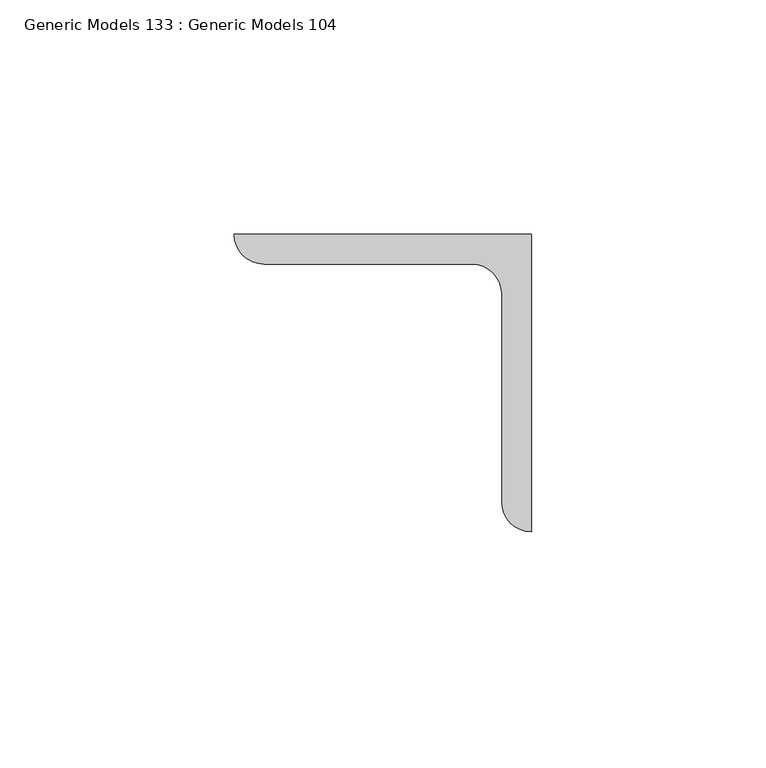
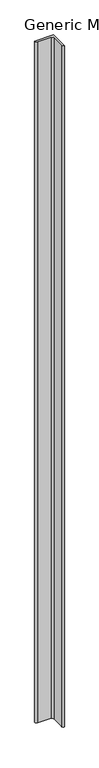
"""IFC4 building model written with IfcOpenShell, lengths in millimetres: proxy geometry, Generic Models 133 : Generic Models 104."""

import ifcopenshell
import ifcopenshell.guid

model = None  # the IFC model being written
_history = None  # IfcOwnerHistory: only IFC2X3 demands one
_inside = {}  # id of a spatial element -> (the spatial element, [elements in it])
_under = {}  # id of a project, library or spatial element -> (it, [spatial elements below it])
_declared = {}  # id of a project -> (the project, [libraries it declares])
_typed = {}  # id of a type object -> (the type object, [elements of that type])
_made_of = {}  # id of a material, layer set ... -> (it, [elements and type objects made of it])


def new_model(schema):
    """Start an empty IFC model of exactly this schema.

    Asked for "IFC4X3", IfcOpenShell would pick the latest addendum, in which some entities
    have other attributes; the version numbers below select the first issue.
    IFC2X3 requires an IfcOwnerHistory on every rooted entity: one is made here for all.
    """
    global model, _history
    if schema == "IFC4X3":
        model = ifcopenshell.file(schema_version=(4, 3, 0, 0))
    else:
        model = ifcopenshell.file(schema=schema)
    _inside.clear()
    _under.clear()
    _declared.clear()
    _typed.clear()
    _made_of.clear()
    _history = None
    if model.schema == "IFC2X3":
        org = make("IfcOrganization", Name="unknown")
        user = make(
            "IfcPersonAndOrganization",
            ThePerson=make("IfcPerson", FamilyName="unknown"),
            TheOrganization=org,
        )
        app = make(
            "IfcApplication",
            ApplicationDeveloper=org,
            Version="unknown",
            ApplicationFullName="unknown",
            ApplicationIdentifier="unknown",
        )
        _history = make(
            "IfcOwnerHistory",
            OwningUser=user,
            OwningApplication=app,
            ChangeAction="ADDED",
            CreationDate=0,
        )
    return model


def make(cls, **values):
    """One entity of the class cls with the attributes given. An attribute that is None is left unset."""
    return model.create_entity(
        cls, **{name: value for name, value in values.items() if value is not None}
    )


def rooted(cls, **values):
    """An entity with a GlobalId (a new one), such as an element, a storey or a relation."""
    return make(cls, GlobalId=ifcopenshell.guid.new(), OwnerHistory=_history, **values)


def si_unit(unit_type, name, prefix=None):
    """IfcSIUnit, for example si_unit("LENGTHUNIT", "METRE", prefix="MILLI")."""
    return make("IfcSIUnit", UnitType=unit_type, Prefix=prefix, Name=name)


def assignment(units):
    """IfcUnitAssignment: the units of a project."""
    return None if units is None else make("IfcUnitAssignment", Units=units)


def point(xyz):
    """IfcCartesianPoint."""
    return None if xyz is None else make("IfcCartesianPoint", Coordinates=xyz)


def direction(xyz):
    """IfcDirection."""
    return None if xyz is None else make("IfcDirection", DirectionRatios=xyz)


def frame(location, z_axis=None, x_axis=None):
    """IfcAxis2Placement3D, a coordinate frame: its origin and axes. An axis left out is left unset."""
    return make(
        "IfcAxis2Placement3D",
        Location=point(location),
        Axis=direction(z_axis),
        RefDirection=direction(x_axis),
    )


def frame_2d(location, x_axis=None):
    """IfcAxis2Placement2D, a coordinate frame in the plane: its origin and x axis."""
    return make(
        "IfcAxis2Placement2D", Location=point(location), RefDirection=direction(x_axis)
    )


def origin():
    """The frame at (0, 0, 0) with its axes left unset."""
    return frame((0.0, 0.0, 0.0))


def place(relative_to, where):
    """IfcLocalPlacement: puts the frame where relative to a parent placement (None: the world)."""
    return make(
        "IfcLocalPlacement", PlacementRelTo=relative_to, RelativePlacement=where
    )


def context(
    kind, dimensions, precision=None, world=None, true_north=None, identifier=None
):
    """IfcGeometricRepresentationContext, for example the 3D "Model" context."""
    return make(
        "IfcGeometricRepresentationContext",
        ContextIdentifier=identifier,
        ContextType=kind,
        CoordinateSpaceDimension=dimensions,
        Precision=precision,
        WorldCoordinateSystem=world,
        TrueNorth=true_north,
    )


def project(units=None, contexts=None):
    """IfcProject with its units and contexts."""
    return rooted(
        "IfcProject",
        Name="project",
        RepresentationContexts=contexts,
        UnitsInContext=assignment(units),
    )


def spatial(cls, under=None, at=None, **own):
    """A site, building, storey or space (cls), placed at a placement, below another one or the project."""
    s = rooted(cls, ObjectPlacement=at, **own)
    if under is not None:
        _under.setdefault(under.id(), (under, []))[1].append(s)
    return s


def polyline(points):
    """IfcPolyline through the points."""
    return make("IfcPolyline", Points=[point(p) for p in points])


def circle_curve(where, radius):
    """IfcCircle in the frame where."""
    return make("IfcCircle", Position=where, Radius=radius)


def trimmed(basis, trim1, trim2, sense, master):
    """IfcTrimmedCurve: the piece of a basis curve between two trims."""
    return make(
        "IfcTrimmedCurve",
        BasisCurve=basis,
        Trim1=trim1,
        Trim2=trim2,
        SenseAgreement=sense,
        MasterRepresentation=master,
    )


def segment(curve, same_sense, transition):
    """IfcCompositeCurveSegment."""
    return make(
        "IfcCompositeCurveSegment",
        Transition=transition,
        SameSense=same_sense,
        ParentCurve=curve,
    )


def composite_curve(segments, self_intersect=None):
    """IfcCompositeCurve: segments joined end to end."""
    return make("IfcCompositeCurve", Segments=segments, SelfIntersect=self_intersect)


def outline(outer, holes=None, kind="AREA"):
    """IfcArbitraryClosedProfileDef: a profile drawn as a closed curve; with holes, ...WithVoids."""
    if holes is None:
        return make("IfcArbitraryClosedProfileDef", ProfileType=kind, OuterCurve=outer)
    return make(
        "IfcArbitraryProfileDefWithVoids",
        ProfileType=kind,
        OuterCurve=outer,
        InnerCurves=holes,
    )


def extrude(swept, where, along, depth):
    """IfcExtrudedAreaSolid: the profile swept, set in the frame where, extruded along a direction by depth."""
    return make(
        "IfcExtrudedAreaSolid",
        SweptArea=swept,
        Position=where,
        ExtrudedDirection=direction(along),
        Depth=depth,
    )


def shape(context_of_items, identifier, shape_type, items):
    """IfcShapeRepresentation: the items that make up one representation, for example the "Body"."""
    return make(
        "IfcShapeRepresentation",
        ContextOfItems=context_of_items,
        RepresentationIdentifier=identifier,
        RepresentationType=shape_type,
        Items=items,
    )


def source(mapping_origin, context_of_items, identifier, shape_type, items):
    """IfcRepresentationMap: a shape defined once, which mapped items show again and again."""
    return make(
        "IfcRepresentationMap",
        MappingOrigin=mapping_origin,
        MappedRepresentation=shape(context_of_items, identifier, shape_type, items),
    )


def transform(
    local_origin,
    x_axis=None,
    y_axis=None,
    z_axis=None,
    scale=None,
    scale2=None,
    scale3=None,
    uniform=True,
):
    """IfcCartesianTransformationOperator3D, or its non-uniform kind. x_axis, y_axis, z_axis: its Axis1, 2, 3."""
    if uniform:
        return make(
            "IfcCartesianTransformationOperator3D",
            Axis1=direction(x_axis),
            Axis2=direction(y_axis),
            LocalOrigin=point(local_origin),
            Scale=scale,
            Axis3=direction(z_axis),
        )
    return make(
        "IfcCartesianTransformationOperator3DnonUniform",
        Axis1=direction(x_axis),
        Axis2=direction(y_axis),
        LocalOrigin=point(local_origin),
        Scale=scale,
        Axis3=direction(z_axis),
        Scale2=scale2,
        Scale3=scale3,
    )


def mapped(mapping_source, mapping_target):
    """IfcMappedItem: shows the shape of a source again, moved by a transform."""
    return make(
        "IfcMappedItem", MappingSource=mapping_source, MappingTarget=mapping_target
    )


def made_of(thing, what):
    """Note that an element or type object is made of a material, layer set ...; save() writes the relation."""
    if what is not None:
        _made_of.setdefault(what.id(), (what, []))[1].append(thing)
    return thing


def element(
    cls,
    number,
    at=None,
    inside=None,
    cuts=None,
    type_object=None,
    material=None,
    context=None,
    identifier="Body",
    shape_type=None,
    held_by="IfcProductDefinitionShape",
    body=None,
    shapes=None,
    **own,
):
    """One element of the class cls, such as IfcWall. Its Tag is "e" and its number.

    at: its placement. inside: the storey or other place that contains it. cuts: it is an
    opening in that element (IfcRelVoidsElement). A single representation is given by context,
    identifier, shape_type and body (its items); several are given by shapes. held_by: the class
    of the entity that holds the representations. save() writes the other relations.
    """
    e = rooted(cls, Tag="e%d" % number, ObjectPlacement=at, **own)
    if body is not None:
        shapes = [shape(context, identifier, shape_type, body)]
    if shapes is not None:
        e.Representation = make(held_by, Representations=shapes)
    if inside is not None:
        _inside.setdefault(inside.id(), (inside, []))[1].append(e)
    if cuts is not None:
        rooted(
            "IfcRelVoidsElement", RelatingBuildingElement=cuts, RelatedOpeningElement=e
        )
    if type_object is not None:
        _typed.setdefault(type_object.id(), (type_object, []))[1].append(e)
    return made_of(e, material)


def aggregate(whole, parts):
    """IfcRelAggregates: a whole, such as a stair, and the parts it consists of."""
    return rooted("IfcRelAggregates", RelatingObject=whole, RelatedObjects=parts)


def save(model, path):
    """Write the relations noted so far, then the file.

    IfcRelAggregates (storeys below a building ...), IfcRelContainedInSpatialStructure (elements
    in a storey), IfcRelDefinesByType, IfcRelAssociatesMaterial and IfcRelDeclares: one each for
    every whole, place, type object, material and project.
    """
    for whole, parts in _under.values():
        aggregate(whole, parts)
    for where, things in _inside.values():
        rooted(
            "IfcRelContainedInSpatialStructure",
            RelatedElements=things,
            RelatingStructure=where,
        )
    for kind, things in _typed.values():
        rooted("IfcRelDefinesByType", RelatedObjects=things, RelatingType=kind)
    for what, things in _made_of.values():
        rooted("IfcRelAssociatesMaterial", RelatedObjects=things, RelatingMaterial=what)
    for by, libraries in _declared.values():
        rooted("IfcRelDeclares", RelatingContext=by, RelatedDefinitions=libraries)
    model.write(path)


def generic_models_133_generic_models_104_530fd59e(model_context):
    return source(origin(), model_context, "Body", "SweptSolid", [
        extrude(outline(composite_curve([segment(polyline([(33377.1840778, 41071.1196612), (33377.1840778, 41007.6196612)]), True, "CONTINUOUS"), segment(trimmed(circle_curve(frame_2d((33377.1840778, 41013.9696612)), 6.35), [point((33377.1840778, 41007.6196612))], [point((33370.8340778, 41013.9696612))], False, "CARTESIAN"), True, "CONTINUOUS"), segment(polyline([(33370.8340778, 41013.9696612), (33370.8340778, 41058.4196612)]), True, "CONTINUOUS"), segment(trimmed(circle_curve(frame_2d((33364.4840778, 41058.4196612)), 6.35), [point((33370.8340778, 41058.4196612))], [point((33364.4840778, 41064.7696612))], True, "CARTESIAN"), True, "CONTINUOUS"), segment(polyline([(33364.4840778, 41064.7696612), (33320.0340778, 41064.7696612)]), True, "CONTINUOUS"), segment(trimmed(circle_curve(frame_2d((33320.0340778, 41071.1196612)), 6.35), [point((33320.0340778, 41064.7696612))], [point((33313.6840778, 41071.1196612))], False, "CARTESIAN"), True, "CONTINUOUS"), segment(polyline([(33313.6840778, 41071.1196612), (33377.1840778, 41071.1196612)]), True, "CONTINUOUS")], self_intersect=False)), frame((0.0, 0.0, 266407.9), z_axis=(0.0, 0.0, 1.0), x_axis=(1.0, 0.0, 0.0)), (0.0, 0.0, 1.0), 2432.1044757),
    ])


if __name__ == "__main__":
    model = new_model("IFC4")
    model_context = context("Model", 3, world=origin())
    ifc_project = project(units=[si_unit("LENGTHUNIT", "METRE", prefix="MILLI")], contexts=[model_context])
    site = spatial("IfcSite", under=ifc_project)
    building = spatial("IfcBuilding", under=site)
    placement = place(None, origin())
    generic_models_133_generic_models_104_shape = generic_models_133_generic_models_104_530fd59e(model_context)
    element("IfcBuildingElementProxy", 1, Name="Generic Models 133 : Generic Models 104", ObjectType="Generic Models 133 : Generic Models 104", at=placement, inside=building, context=model_context, shape_type="MappedRepresentation", body=[
        mapped(generic_models_133_generic_models_104_shape, transform((0.0, 0.0, 0.0), x_axis=(1.0, 0.0, 0.0), y_axis=(0.0, 1.0, 0.0), z_axis=(0.0, 0.0, 1.0))),
    ])
    save(model, "model.ifc")

# Revit data of these elements
# Element 1 (IfcBuildingElementProxy, "Generic Models 133 : Generic Models 104")
#   Materials on its faces: "(2) BACK/BACK GALVANIZED ANGLES (2) L2 1/2 X 2 1/2 X 1/4\")"
# Materials
#   "(2) BACK/BACK GALVANIZED ANGLES (2) L2 1/2 X 2 1/2 X 1/4\")": class "Unassigned", colour RGB 211 211 211, transparency 0, Cost = 0
